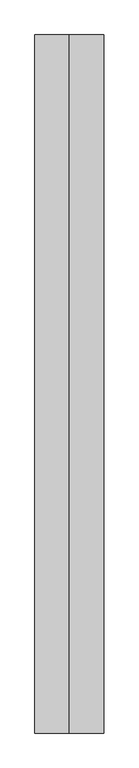
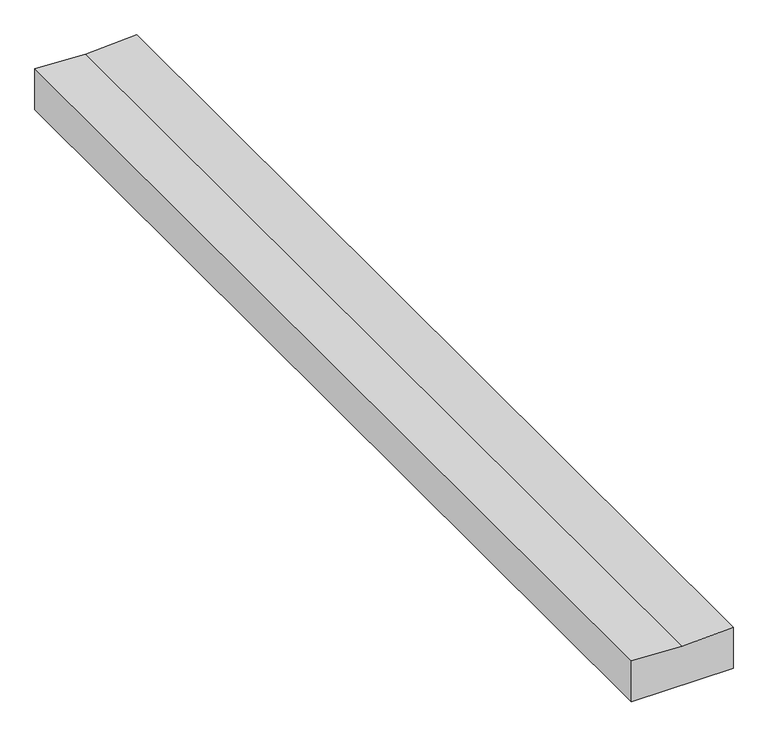
"""IFC4 building model written with IfcOpenShell, lengths in millimetres: proxy geometry, FIRESTONE INSULATION002 : FIRESTONE INSULATION002."""

from ifc_helpers import new_model, si_unit, frame, origin, place, context, project, spatial, polyline, outline, extrude, source, transform, mapped, element, save


def generic_models_d8f1048d(model_context):
    return source(origin(), model_context, "Body", "SweptSolid", [
        extrude(outline(polyline([(40131.746, -4797.9038825), (40131.746, -4601.0538825), (40216.0142809, -4601.0538825), (40211.0127094, -4699.8063764), (40216.0142809, -4797.9038825), (40131.746, -4797.9038825)])), frame((0.0, -1052.6406573, 0.0), z_axis=(0.0, 1.0, 0.0), x_axis=(0.0, 0.0, 1.0)), (0.0, 0.0, 1.0), 2000.0),
    ])


if __name__ == "__main__":
    model = new_model("IFC4")
    model_context = context("Model", 3, world=origin())
    ifc_project = project(units=[si_unit("LENGTHUNIT", "METRE", prefix="MILLI")], contexts=[model_context])
    site = spatial("IfcSite", under=ifc_project)
    building = spatial("IfcBuilding", under=site)
    placement = place(None, origin())
    generic_models_shape = generic_models_d8f1048d(model_context)
    element("IfcBuildingElementProxy", 1, Name="FIRESTONE INSULATION002 : FIRESTONE INSULATION002", ObjectType="FIRESTONE INSULATION002 : FIRESTONE INSULATION002", at=placement, inside=building, context=model_context, shape_type="MappedRepresentation", body=[
        mapped(generic_models_shape, transform((0.0, 0.0, 0.0), x_axis=(1.0, 0.0, 0.0), y_axis=(0.0, 1.0, 0.0), z_axis=(0.0, 0.0, 1.0))),
    ])
    save(model, "model.ifc")

# Revit data of these elements
# Type "FIRESTONE INSULATION002 : FIRESTONE INSULATION002"
#   NameOverride = "FIRESTONE INSULATION002"
# Element 1 (IfcBuildingElementProxy, "FIRESTONE INSULATION002 : FIRESTONE INSULATION002")
#   Materials on its faces: "TAPERED 2X SLEEPERS - SLOPED TO DRAIN"
# Materials
#   "TAPERED 2X SLEEPERS - SLOPED TO DRAIN": class "Unassigned", colour RGB 234 198 178, transparency 0
